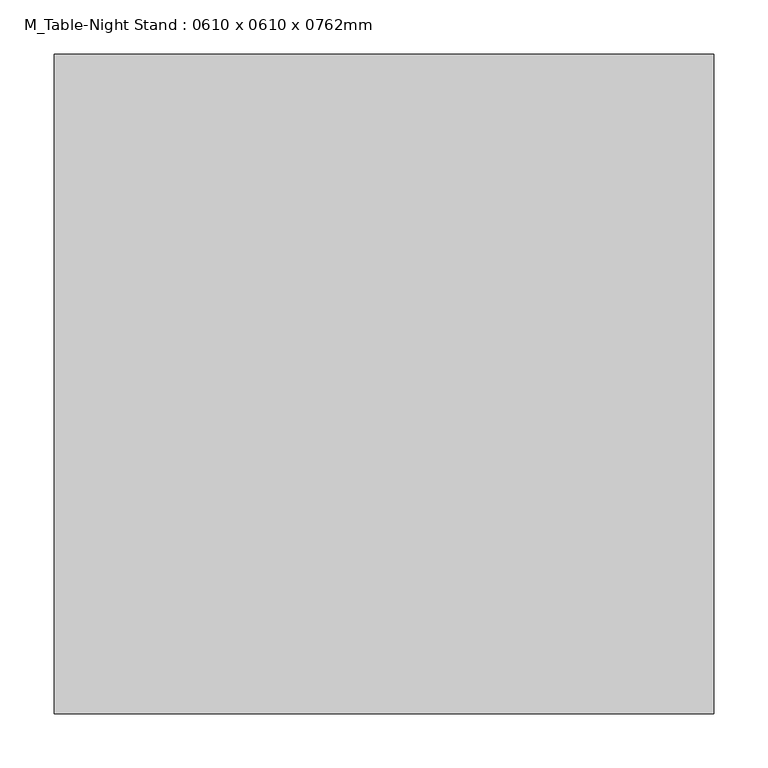
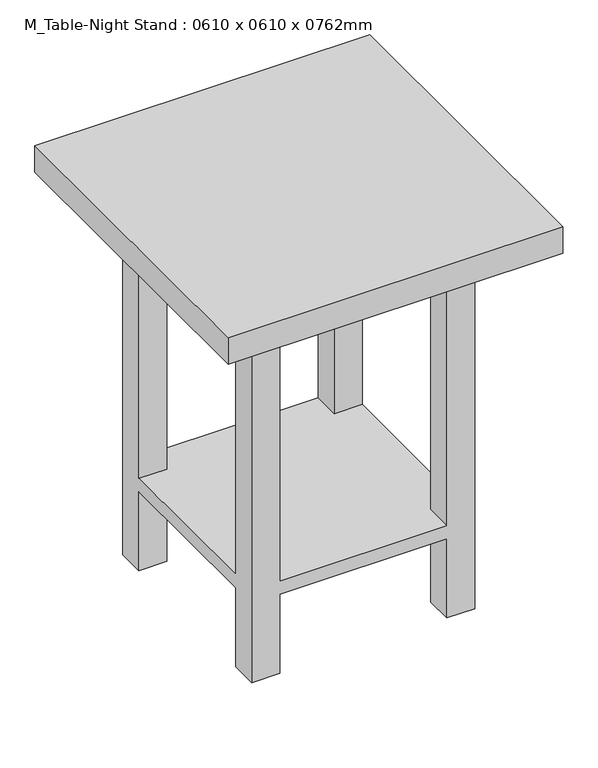
"""IFC4 building model written with IfcOpenShell, lengths in millimetres: furniture geometry, M_Table-Night Stand : 0610 x 0610 x 0762mm."""

from ifc_helpers import new_model, si_unit, frame, origin, place, context, project, spatial, polyline, outline, extrude, faceted_brep, source, transform, mapped, element, save


def m_table_night_stand_0610_x_0610_x_0762mm_a39a3fb5(model_context):
    return source(origin(), model_context, "Body", "SolidModel", [
        faceted_brep([(156.1336303, 508.4, 711.2), (105.3336303, 508.4, 711.2), (105.3336303, 457.6, 711.2), (156.1336303, 457.6, 711.2), (156.1336303, 152.4, 711.2), (105.3336303, 152.4, 711.2), (105.3336303, 101.6, 711.2), (156.1336303, 101.6, 711.2), (512.1336303, 508.4, 711.2), (461.3336303, 508.4, 711.2), (461.3336303, 457.6, 711.2), (512.1336303, 457.6, 711.2), (512.1336303, 152.4, 711.2), (461.3336303, 152.4, 711.2), (461.3336303, 101.6, 711.2), (512.1336303, 101.6, 711.2), (156.1336303, 508.4, 0.0), (156.1336303, 457.6, 0.0), (105.3336303, 457.6, 0.0), (105.3336303, 508.4, 0.0), (156.1336303, 152.4, 0.0), (156.1336303, 101.6, 0.0), (105.3336303, 101.6, 0.0), (105.3336303, 152.4, 0.0), (512.1336303, 508.4, 0.0), (512.1336303, 457.6, 0.0), (461.3336303, 457.6, 0.0), (461.3336303, 508.4, 0.0), (512.1336303, 152.4, 0.0), (512.1336303, 101.6, 0.0), (461.3336303, 101.6, 0.0), (461.3336303, 152.4, 0.0), (156.1336303, 508.4, 177.8), (461.3336303, 508.4, 177.8), (461.3336303, 508.4, 152.4), (156.1336303, 508.4, 152.4), (105.3336303, 457.6, 152.4), (105.3336303, 152.4, 152.4), (105.3336303, 152.4, 177.8), (105.3336303, 457.6, 177.8), (156.1336303, 457.6, 177.8), (156.1336303, 457.6, 152.4), (156.1336303, 152.4, 177.8), (156.1336303, 152.4, 152.4), (156.1336303, 101.6, 152.4), (461.3336303, 101.6, 152.4), (461.3336303, 101.6, 177.8), (156.1336303, 101.6, 177.8), (461.3336303, 457.6, 177.8), (461.3336303, 457.6, 152.4), (512.1336303, 457.6, 177.8), (512.1336303, 457.6, 152.4), (512.1336303, 152.4, 177.8), (512.1336303, 152.4, 152.4), (461.3336303, 152.4, 177.8), (461.3336303, 152.4, 152.4)], [[[0, 1, 2, 3]], [[4, 5, 6, 7]], [[8, 9, 10, 11]], [[12, 13, 14, 15]], [[16, 17, 18, 19]], [[20, 21, 22, 23]], [[24, 25, 26, 27]], [[28, 29, 30, 31]], [[1, 0, 32, 33, 9, 8, 24, 27, 34, 35, 16, 19]], [[2, 1, 19, 18, 36, 37, 23, 22, 6, 5, 38, 39]], [[3, 2, 39, 40]], [[18, 17, 41, 36]], [[0, 3, 40, 32]], [[17, 16, 35, 41]], [[5, 4, 42, 38]], [[20, 23, 37, 43]], [[7, 6, 22, 21, 44, 45, 30, 29, 15, 14, 46, 47]], [[4, 7, 47, 42]], [[21, 20, 43, 44]], [[10, 9, 33, 48]], [[27, 26, 49, 34]], [[11, 10, 48, 50]], [[26, 25, 51, 49]], [[8, 11, 50, 52, 12, 15, 29, 28, 53, 51, 25, 24]], [[13, 12, 52, 54]], [[28, 31, 55, 53]], [[14, 13, 54, 46]], [[31, 30, 45, 55]], [[39, 38, 42, 47, 46, 54, 52, 50, 48, 33, 32, 40]], [[35, 34, 49, 51, 53, 55, 45, 44, 43, 37, 36, 41]]]),
        extrude(outline(polyline([(613.7336303, 0.0), (3.7336303, 0.0), (3.7336303, 610.0), (613.7336303, 610.0), (613.7336303, 0.0)])), frame((0.0, 0.0, 711.2), z_axis=(0.0, 0.0, 1.0), x_axis=(1.0, 0.0, 0.0)), (0.0, 0.0, 1.0), 50.8),
    ])


if __name__ == "__main__":
    model = new_model("IFC4")
    model_context = context("Model", 3, world=origin())
    ifc_project = project(units=[si_unit("LENGTHUNIT", "METRE", prefix="MILLI")], contexts=[model_context])
    site = spatial("IfcSite", under=ifc_project)
    building = spatial("IfcBuilding", under=site)
    placement = place(None, origin())
    m_table_night_stand_0610_x_0610_x_0762mm_shape = m_table_night_stand_0610_x_0610_x_0762mm_a39a3fb5(model_context)
    element("IfcFurniture", 1, ObjectType="M_Table-Night Stand : 0610 x 0610 x 0762mm", at=placement, inside=building, context=model_context, shape_type="MappedRepresentation", body=[
        mapped(m_table_night_stand_0610_x_0610_x_0762mm_shape, transform((0.0, 0.0, 0.0), x_axis=(1.0, 0.0, 0.0), y_axis=(0.0, 1.0, 0.0), z_axis=(0.0, 0.0, 1.0))),
    ])
    save(model, "model.ifc")

# Revit data of these elements
# Type "M_Table-Night Stand : 0610 x 0610 x 0762mm"
#   Depth = 0.61 m
#   Height = 0.762 m
#   Width = 0.61 m
#   Base Material = Birch
#   Top Material = Laminate, Ivory, Matte
# Element 1 (IfcFurniture, "M_Table-Night Stand : 0610 x 0610 x 0762mm")
#   Materials on its faces: "Birch", "Laminate, Ivory, Matte"
# Materials
#   "Birch": class "Wood", colour RGB 224 178 126, transparency 0, Description = "Betula Alleghaniensis", Cost = 0
#   "Laminate, Ivory, Matte": class "Plastic", colour RGB 247 247 229, transparency 0, Description = "Plastic Laminate - Ivory, Matte", Cost = 0
